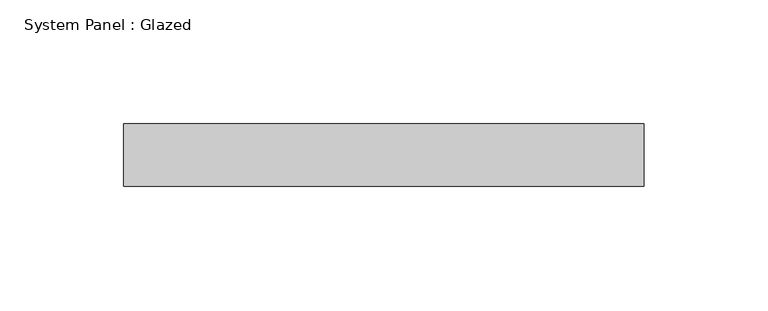
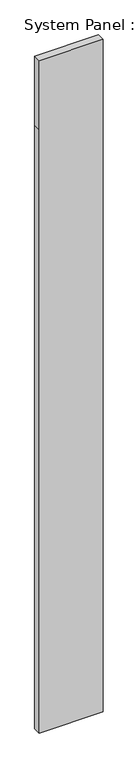
"""IFC4 building model written with IfcOpenShell, lengths in millimetres: plate geometry, System Panel : Glazed."""

from ifc_helpers import new_model, si_unit, frame, origin, place, context, project, spatial, polyline, outline, extrude, source, transform, mapped, element, save


def system_panel_glazed_4de51809(model_context):
    return source(origin(), model_context, "Body", "SweptSolid", [
        extrude(outline(polyline([(0.0, -105.4575643), (0.0, 105.4575643), (2101.85, 105.4575643), (2343.15, 105.4575643), (2343.15, -105.4575643), (2101.85, -105.4575643), (0.0, -105.4575643)])), frame((0.0, 19.05, 0.0), z_axis=(0.0, 1.0, 0.0), x_axis=(0.0, 0.0, 1.0)), (0.0, 0.0, 1.0), 25.4),
    ])


if __name__ == "__main__":
    model = new_model("IFC4")
    model_context = context("Model", 3, world=origin())
    ifc_project = project(units=[si_unit("LENGTHUNIT", "METRE", prefix="MILLI")], contexts=[model_context])
    site = spatial("IfcSite", under=ifc_project)
    building = spatial("IfcBuilding", under=site)
    placement = place(None, origin())
    system_panel_glazed_shape = system_panel_glazed_4de51809(model_context)
    element("IfcPlate", 1, ObjectType="System Panel : Glazed", at=placement, inside=building, context=model_context, shape_type="MappedRepresentation", body=[
        mapped(system_panel_glazed_shape, transform((0.0, 0.0, 0.0), x_axis=(1.0, 0.0, 0.0), y_axis=(0.0, 1.0, 0.0), z_axis=(0.0, 0.0, 1.0))),
    ])
    save(model, "model.ifc")

# Revit data of these elements
# Element 1 (IfcPlate, "System Panel : Glazed")
#   Materials on its faces: "Glass"
# Materials
#   "Glass": class "Glass", colour RGB 0 128 192, transparency 0.75
